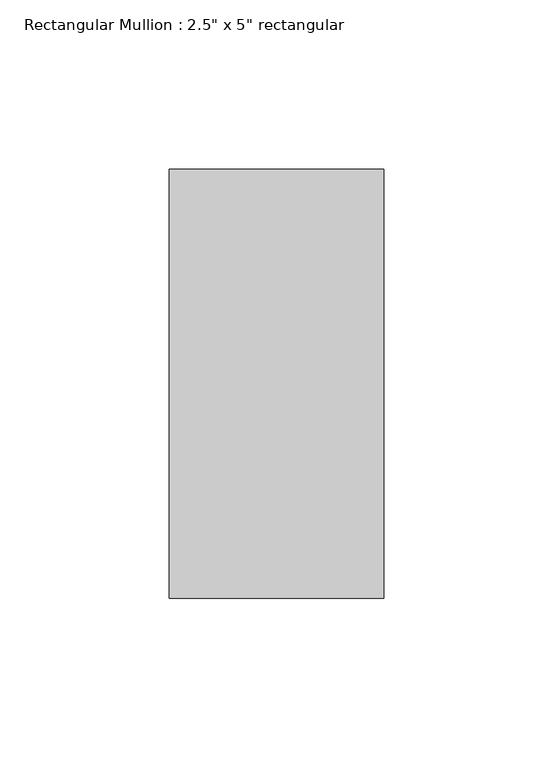
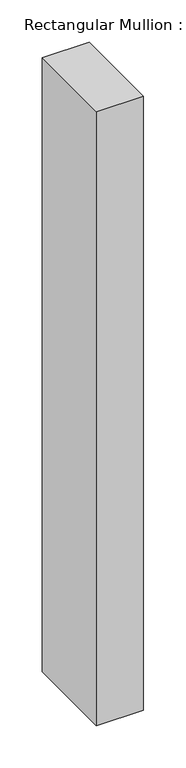
"""IFC4 building model written with IfcOpenShell, lengths in millimetres: member geometry."""

import ifcopenshell
import ifcopenshell.guid

model = None  # the IFC model being written
_history = None  # IfcOwnerHistory: only IFC2X3 demands one
_inside = {}  # id of a spatial element -> (the spatial element, [elements in it])
_under = {}  # id of a project, library or spatial element -> (it, [spatial elements below it])
_declared = {}  # id of a project -> (the project, [libraries it declares])
_typed = {}  # id of a type object -> (the type object, [elements of that type])
_made_of = {}  # id of a material, layer set ... -> (it, [elements and type objects made of it])


def new_model(schema):
    """Start an empty IFC model of exactly this schema.

    Asked for "IFC4X3", IfcOpenShell would pick the latest addendum, in which some entities
    have other attributes; the version numbers below select the first issue.
    IFC2X3 requires an IfcOwnerHistory on every rooted entity: one is made here for all.
    """
    global model, _history
    if schema == "IFC4X3":
        model = ifcopenshell.file(schema_version=(4, 3, 0, 0))
    else:
        model = ifcopenshell.file(schema=schema)
    _inside.clear()
    _under.clear()
    _declared.clear()
    _typed.clear()
    _made_of.clear()
    _history = None
    if model.schema == "IFC2X3":
        org = make("IfcOrganization", Name="unknown")
        user = make(
            "IfcPersonAndOrganization",
            ThePerson=make("IfcPerson", FamilyName="unknown"),
            TheOrganization=org,
        )
        app = make(
            "IfcApplication",
            ApplicationDeveloper=org,
            Version="unknown",
            ApplicationFullName="unknown",
            ApplicationIdentifier="unknown",
        )
        _history = make(
            "IfcOwnerHistory",
            OwningUser=user,
            OwningApplication=app,
            ChangeAction="ADDED",
            CreationDate=0,
        )
    return model


def make(cls, **values):
    """One entity of the class cls with the attributes given. An attribute that is None is left unset."""
    return model.create_entity(
        cls, **{name: value for name, value in values.items() if value is not None}
    )


def rooted(cls, **values):
    """An entity with a GlobalId (a new one), such as an element, a storey or a relation."""
    return make(cls, GlobalId=ifcopenshell.guid.new(), OwnerHistory=_history, **values)


def si_unit(unit_type, name, prefix=None):
    """IfcSIUnit, for example si_unit("LENGTHUNIT", "METRE", prefix="MILLI")."""
    return make("IfcSIUnit", UnitType=unit_type, Prefix=prefix, Name=name)


def assignment(units):
    """IfcUnitAssignment: the units of a project."""
    return None if units is None else make("IfcUnitAssignment", Units=units)


def point(xyz):
    """IfcCartesianPoint."""
    return None if xyz is None else make("IfcCartesianPoint", Coordinates=xyz)


def direction(xyz):
    """IfcDirection."""
    return None if xyz is None else make("IfcDirection", DirectionRatios=xyz)


def frame(location, z_axis=None, x_axis=None):
    """IfcAxis2Placement3D, a coordinate frame: its origin and axes. An axis left out is left unset."""
    return make(
        "IfcAxis2Placement3D",
        Location=point(location),
        Axis=direction(z_axis),
        RefDirection=direction(x_axis),
    )


def origin():
    """The frame at (0, 0, 0) with its axes left unset."""
    return frame((0.0, 0.0, 0.0))


def place(relative_to, where):
    """IfcLocalPlacement: puts the frame where relative to a parent placement (None: the world)."""
    return make(
        "IfcLocalPlacement", PlacementRelTo=relative_to, RelativePlacement=where
    )


def context(
    kind, dimensions, precision=None, world=None, true_north=None, identifier=None
):
    """IfcGeometricRepresentationContext, for example the 3D "Model" context."""
    return make(
        "IfcGeometricRepresentationContext",
        ContextIdentifier=identifier,
        ContextType=kind,
        CoordinateSpaceDimension=dimensions,
        Precision=precision,
        WorldCoordinateSystem=world,
        TrueNorth=true_north,
    )


def project(units=None, contexts=None):
    """IfcProject with its units and contexts."""
    return rooted(
        "IfcProject",
        Name="project",
        RepresentationContexts=contexts,
        UnitsInContext=assignment(units),
    )


def spatial(cls, under=None, at=None, **own):
    """A site, building, storey or space (cls), placed at a placement, below another one or the project."""
    s = rooted(cls, ObjectPlacement=at, **own)
    if under is not None:
        _under.setdefault(under.id(), (under, []))[1].append(s)
    return s


def polyline(points):
    """IfcPolyline through the points."""
    return make("IfcPolyline", Points=[point(p) for p in points])


def outline(outer, holes=None, kind="AREA"):
    """IfcArbitraryClosedProfileDef: a profile drawn as a closed curve; with holes, ...WithVoids."""
    if holes is None:
        return make("IfcArbitraryClosedProfileDef", ProfileType=kind, OuterCurve=outer)
    return make(
        "IfcArbitraryProfileDefWithVoids",
        ProfileType=kind,
        OuterCurve=outer,
        InnerCurves=holes,
    )


def extrude(swept, where, along, depth):
    """IfcExtrudedAreaSolid: the profile swept, set in the frame where, extruded along a direction by depth."""
    return make(
        "IfcExtrudedAreaSolid",
        SweptArea=swept,
        Position=where,
        ExtrudedDirection=direction(along),
        Depth=depth,
    )


def shape(context_of_items, identifier, shape_type, items):
    """IfcShapeRepresentation: the items that make up one representation, for example the "Body"."""
    return make(
        "IfcShapeRepresentation",
        ContextOfItems=context_of_items,
        RepresentationIdentifier=identifier,
        RepresentationType=shape_type,
        Items=items,
    )


def source(mapping_origin, context_of_items, identifier, shape_type, items):
    """IfcRepresentationMap: a shape defined once, which mapped items show again and again."""
    return make(
        "IfcRepresentationMap",
        MappingOrigin=mapping_origin,
        MappedRepresentation=shape(context_of_items, identifier, shape_type, items),
    )


def transform(
    local_origin,
    x_axis=None,
    y_axis=None,
    z_axis=None,
    scale=None,
    scale2=None,
    scale3=None,
    uniform=True,
):
    """IfcCartesianTransformationOperator3D, or its non-uniform kind. x_axis, y_axis, z_axis: its Axis1, 2, 3."""
    if uniform:
        return make(
            "IfcCartesianTransformationOperator3D",
            Axis1=direction(x_axis),
            Axis2=direction(y_axis),
            LocalOrigin=point(local_origin),
            Scale=scale,
            Axis3=direction(z_axis),
        )
    return make(
        "IfcCartesianTransformationOperator3DnonUniform",
        Axis1=direction(x_axis),
        Axis2=direction(y_axis),
        LocalOrigin=point(local_origin),
        Scale=scale,
        Axis3=direction(z_axis),
        Scale2=scale2,
        Scale3=scale3,
    )


def mapped(mapping_source, mapping_target):
    """IfcMappedItem: shows the shape of a source again, moved by a transform."""
    return make(
        "IfcMappedItem", MappingSource=mapping_source, MappingTarget=mapping_target
    )


def made_of(thing, what):
    """Note that an element or type object is made of a material, layer set ...; save() writes the relation."""
    if what is not None:
        _made_of.setdefault(what.id(), (what, []))[1].append(thing)
    return thing


def element(
    cls,
    number,
    at=None,
    inside=None,
    cuts=None,
    type_object=None,
    material=None,
    context=None,
    identifier="Body",
    shape_type=None,
    held_by="IfcProductDefinitionShape",
    body=None,
    shapes=None,
    **own,
):
    """One element of the class cls, such as IfcWall. Its Tag is "e" and its number.

    at: its placement. inside: the storey or other place that contains it. cuts: it is an
    opening in that element (IfcRelVoidsElement). A single representation is given by context,
    identifier, shape_type and body (its items); several are given by shapes. held_by: the class
    of the entity that holds the representations. save() writes the other relations.
    """
    e = rooted(cls, Tag="e%d" % number, ObjectPlacement=at, **own)
    if body is not None:
        shapes = [shape(context, identifier, shape_type, body)]
    if shapes is not None:
        e.Representation = make(held_by, Representations=shapes)
    if inside is not None:
        _inside.setdefault(inside.id(), (inside, []))[1].append(e)
    if cuts is not None:
        rooted(
            "IfcRelVoidsElement", RelatingBuildingElement=cuts, RelatedOpeningElement=e
        )
    if type_object is not None:
        _typed.setdefault(type_object.id(), (type_object, []))[1].append(e)
    return made_of(e, material)


def aggregate(whole, parts):
    """IfcRelAggregates: a whole, such as a stair, and the parts it consists of."""
    return rooted("IfcRelAggregates", RelatingObject=whole, RelatedObjects=parts)


def save(model, path):
    """Write the relations noted so far, then the file.

    IfcRelAggregates (storeys below a building ...), IfcRelContainedInSpatialStructure (elements
    in a storey), IfcRelDefinesByType, IfcRelAssociatesMaterial and IfcRelDeclares: one each for
    every whole, place, type object, material and project.
    """
    for whole, parts in _under.values():
        aggregate(whole, parts)
    for where, things in _inside.values():
        rooted(
            "IfcRelContainedInSpatialStructure",
            RelatedElements=things,
            RelatingStructure=where,
        )
    for kind, things in _typed.values():
        rooted("IfcRelDefinesByType", RelatedObjects=things, RelatingType=kind)
    for what, things in _made_of.values():
        rooted("IfcRelAssociatesMaterial", RelatedObjects=things, RelatingMaterial=what)
    for by, libraries in _declared.values():
        rooted("IfcRelDeclares", RelatingContext=by, RelatedDefinitions=libraries)
    model.write(path)


def member_049a2e78(model_context):
    return source(origin(), model_context, "Body", "SweptSolid", [
        extrude(outline(polyline([(31.75, 63.5), (31.75, -63.5), (-31.75, -63.5), (-31.75, 63.5), (31.75, 63.5)])), frame((0.0, 0.0, -882.65), z_axis=(0.0, 0.0, 1.0), x_axis=(1.0, 0.0, 0.0)), (0.0, 0.0, 1.0), 882.65),
    ])


if __name__ == "__main__":
    model = new_model("IFC4")
    model_context = context("Model", 3, world=origin())
    ifc_project = project(units=[si_unit("LENGTHUNIT", "METRE", prefix="MILLI")], contexts=[model_context])
    site = spatial("IfcSite", under=ifc_project)
    building = spatial("IfcBuilding", under=site)
    placement = place(None, origin())
    member_shape = member_049a2e78(model_context)
    element("IfcMember", 1, ObjectType="Rectangular Mullion : 2.5\" x 5\" rectangular", at=placement, inside=building, context=model_context, shape_type="MappedRepresentation", body=[
        mapped(member_shape, transform((0.0, 0.0, 0.0), x_axis=(1.0, 0.0, 0.0), y_axis=(0.0, 1.0, 0.0), z_axis=(0.0, 0.0, 1.0))),
    ])
    save(model, "model.ifc")

# Revit data of these elements
# Project information
#   Organization Name = "G3B Press"
#   Organization Description = "Paul F. Aubin Cosulting Services, Inc."
#   Building Name = "Revit Essentials for Architecture"
#   Author = "Paul F. Aubin"
#   Author Website = "https://www.paulaubin.com"
#   Copyright = "Copyright © 2020 Paul F Aubin, all rights reserved"
#   Design Option = "Main Model"
#   Project Issue Date = "8/1/2020"
#   Project Status = "Design Development"
#   Client Name = "Families and the Family Editor"
#   Project Address = "123 State ST\nSuite 301\nChicago, IL 60606"
#   Project Name = "11 Commercial"
#   Project Number = "2020.04A"
# Type "Rectangular Mullion : 2.5\" x 5\" rectangular"
#   built-in parameter 1007304 = 0.416667 (stored number, unit not read)
#   built-in parameter 1007301 = 0.104167 (stored number, unit not read)
#   built-in parameter 1007300 = 0.104167 (stored number, unit not read)
# Element 1 (IfcMember, "Rectangular Mullion : 2.5\" x 5\" rectangular")
#   Materials on its faces: "Aluminum"
# Materials
#   "Aluminum": class "Metal", colour RGB 247 247 247, transparency 0, Description = "Aluminum 6061", Cost = 0
